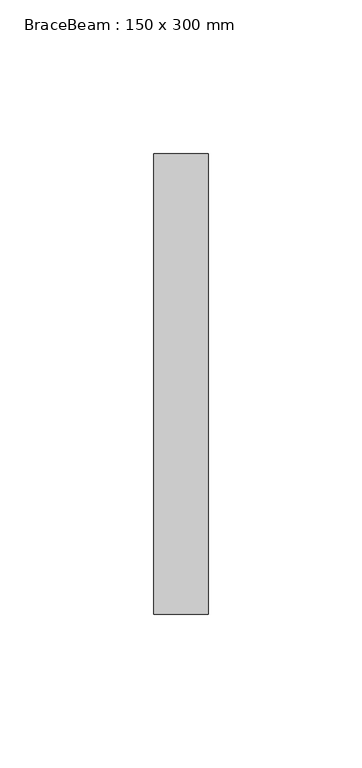
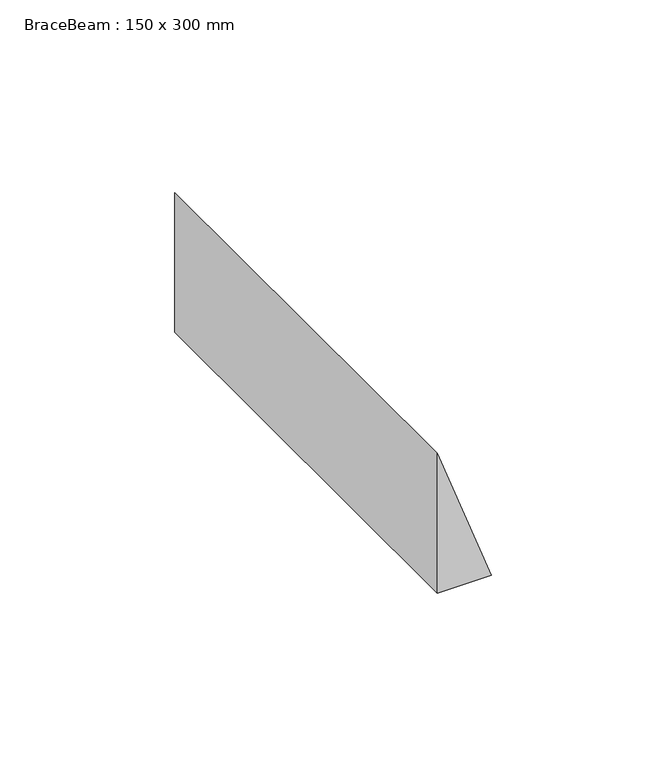
"""IFC4 building model written with IfcOpenShell, lengths in millimetres: beam geometry, BraceBeam : 150 x 300 mm."""

from ifc_helpers import new_model, si_unit, frame, origin, place, context, project, spatial, polyline, outline, extrude, source, transform, mapped, element, save


def bracebeam_150_x_300_mm_686c8613(model_context):
    return source(origin(), model_context, "Body", "SweptSolid", [
        extrude(outline(polyline([(-150.0, 13.6050484), (-150.0, 31.3638209), (-101.2081735, 13.6050484), (-150.0, 13.6050484)])), frame((0.0, -75.0, 0.0), z_axis=(0.0, 1.0, 0.0), x_axis=(0.0, 0.0, 1.0)), (0.0, 0.0, 1.0), 150.0),
    ])


if __name__ == "__main__":
    model = new_model("IFC4")
    model_context = context("Model", 3, world=origin())
    ifc_project = project(units=[si_unit("LENGTHUNIT", "METRE", prefix="MILLI")], contexts=[model_context])
    site = spatial("IfcSite", under=ifc_project)
    building = spatial("IfcBuilding", under=site)
    placement = place(None, origin())
    bracebeam_150_x_300_mm_shape = bracebeam_150_x_300_mm_686c8613(model_context)
    element("IfcBeam", 1, ObjectType="BraceBeam : 150 x 300 mm", at=placement, inside=building, context=model_context, shape_type="MappedRepresentation", body=[
        mapped(bracebeam_150_x_300_mm_shape, transform((0.0, 0.0, 0.0), x_axis=(1.0, 0.0, 0.0), y_axis=(0.0, 1.0, 0.0), z_axis=(0.0, 0.0, 1.0))),
    ])
    save(model, "model.ifc")

# Revit data of these elements
# Type "BraceBeam : 150 x 300 mm"
#   ExpertTruss = "Height\th\r\nWidth\tb"
#   Name [instance default] = ""
#   m [instance default] = 0 mm
#   ip_c_cut_control [instance default] = 1300 mm
#   ip_c_cut [instance default] = 1300 mm
#   h_fix [instance default] = 900 mm
#   d/2 [instance default] = 1750 mm
#   c_cut_incl [instance default] = -1000 mm
#   c_cut [instance default] = 0 mm
#   beta0_2 [instance default] = 90.00°
#   beta0_1 [instance default] = 90.00°
#   alfaMax [instance default] = 0.00°
#   alfa0_2 [instance default] = 90.00°
#   ZOffsetStr_0 [instance default] = 150 mm
#   ZOffsetStr [instance default] = 0 mm
#   ZOffsetEnd_0 [instance default] = 150 mm
#   ZOffsetEnd [instance default] = 0 mm
#   Beta2 [instance default] = 0.00°
#   Beta1 [instance default] = 0.00°
#   Alfa_str [instance default] = 0.00°
#   Alfa_cut_control [instance default] = 90.00°
#   Alfa_cut [instance default] = 90.00°
#   AlfaMAX [instance default] = 0.00°
#   Alfa2_0 [instance default] = 0.00°
#   Alfa2 [instance default] = 0.00°
#   Alfa1_0 [instance default] = 0.00°
#   Alfa1 [instance default] = 0.00°
#   A_max_Str [instance default] = 0.00°
#   h_void [instance default] = 3000 mm
#   beam_L_0 [instance default] = 100 mm
#   beam_L [instance default] = 0 mm
#   b_void [instance default] = 160 mm
#   alfa0_1 [instance default] = 90.00°
#   b = 150 mm
#   YOffsetStr [instance default] = 0 mm
#   YOffsetEnd [instance default] = 0 mm
#   XOffsetStr_0 [instance default] = 3500 mm
#   XOffsetStr [instance default] = 0 mm
#   XOffsetEnd_0 [instance default] = 3500 mm
#   XOffsetEnd [instance default] = 0 mm
#   L_void_0 [instance default] = 100 mm
#   L_void [instance default] = 0 mm
#   E2 [instance default] = 0.00°
#   E1 [instance default] = 0.00°
#   Length [instance default] = 3500 mm
#   h = 300 mm
#   Alfa [instance default] = 0.00°
#   A_max_End [instance default] = 0.00°
#   A_max [instance default] = 0.00°
#   A4 [instance default] = 0.00°
#   A3 [instance default] = 0.00°
#   A2 [instance default] = 0.00°
#   A1 [instance default] = 0.00°
#   BetaAngles [instance default] = no
#   Material [instance default] = Wood Standard
# Element 1 (IfcBeam, "BraceBeam : 150 x 300 mm")
#   d/2 = 104.789 mm
#   beta0_2 = 70.00°
#   alfaMax = -20.00°
#   alfa0_2 = 70.00°
#   AlfaMAX = -20.00°
#   Alfa2_0 = -20.00°
#   Alfa2 = -20.00°
#   h_void = 4091.911 mm
#   beam_L_0 = 873.529 mm
#   beam_L = 873.529 mm
#   XOffsetStr_0 = 59.577 mm
#   XOffsetStr = 150 mm
#   XOffsetEnd_0 = 49.951 mm
#   XOffsetEnd = 159.627 mm
#   L_void_0 = 2064.996 mm
#   L_void = 2064.996 mm
#   Materials on its faces: "Wood Standard"
# Materials
#   "Wood Standard": class "Drewno", colour RGB 196 146 67, transparency 0, Cost = 0
